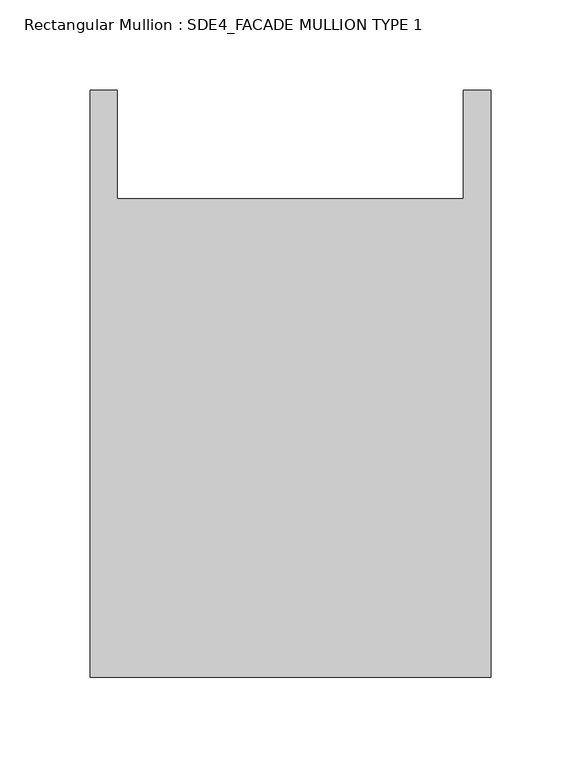
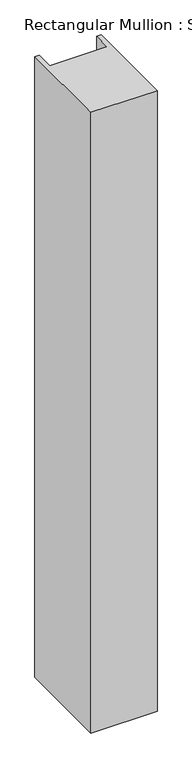
"""IFC4 building model written with IfcOpenShell, lengths in millimetres: member geometry, Rectangular Mullion : SDE4_FACADE MULLION TYPE 1."""

from ifc_helpers import new_model, si_unit, frame, origin, place, context, project, spatial, polyline, outline, extrude, source, transform, mapped, element, save


def rectangular_mullion_sde4_facade_mullion_type_1_accd64c0(model_context):
    return source(origin(), model_context, "Body", "SweptSolid", [
        extrude(outline(polyline([(111.0, -132.5), (-111.0, -132.5), (-111.0, 192.5), (-96.0, 192.5), (-96.0, 132.5), (96.0, 132.5), (96.0, 192.5), (111.0, 192.5), (111.0, -132.5)])), frame((0.0, 0.0, -2200.0), z_axis=(0.0, 0.0, 1.0), x_axis=(1.0, 0.0, 0.0)), (0.0, 0.0, 1.0), 2200.0),
    ])


if __name__ == "__main__":
    model = new_model("IFC4")
    model_context = context("Model", 3, world=origin())
    ifc_project = project(units=[si_unit("LENGTHUNIT", "METRE", prefix="MILLI")], contexts=[model_context])
    site = spatial("IfcSite", under=ifc_project)
    building = spatial("IfcBuilding", under=site)
    placement = place(None, origin())
    rectangular_mullion_sde4_facade_mullion_type_1_shape = rectangular_mullion_sde4_facade_mullion_type_1_accd64c0(model_context)
    element("IfcMember", 1, ObjectType="Rectangular Mullion : SDE4_FACADE MULLION TYPE 1", at=placement, inside=building, context=model_context, shape_type="MappedRepresentation", body=[
        mapped(rectangular_mullion_sde4_facade_mullion_type_1_shape, transform((0.0, 0.0, 0.0), x_axis=(1.0, 0.0, 0.0), y_axis=(0.0, 1.0, 0.0), z_axis=(0.0, 0.0, 1.0))),
    ])
    save(model, "model.ifc")

# Revit data of these elements
# Type "Rectangular Mullion : SDE4_FACADE MULLION TYPE 1"
#   built-in parameter 1007322 = 0.869423 (stored number, unit not read)
#   built-in parameter 1007321 = 0.364173 (stored number, unit not read)
#   built-in parameter 1007320 = 0.364173 (stored number, unit not read)
